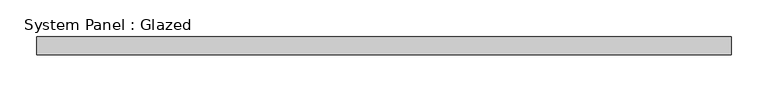
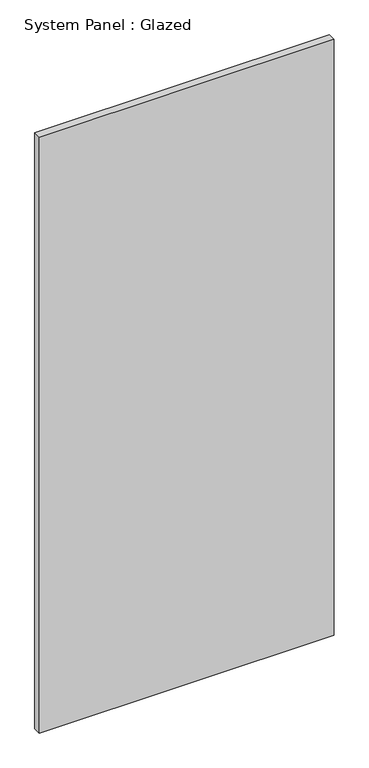
"""IFC4 building model written with IfcOpenShell, lengths in millimetres: plate geometry, System Panel : Glazed."""

from ifc_helpers import new_model, si_unit, origin, origin_with_axes, place, context, project, spatial, polyline, outline, extrude, source, transform, mapped, element, save


def system_panel_glazed_49f26875(model_context):
    return source(origin(), model_context, "Body", "SweptSolid", [
        extrude(outline(polyline([(475.0, 24.5), (-475.0, 24.5), (-475.0, 49.5), (475.0, 49.5), (475.0, 24.5)])), origin_with_axes(), (0.0, 0.0, 1.0), 2030.4462072),
    ])


if __name__ == "__main__":
    model = new_model("IFC4")
    model_context = context("Model", 3, world=origin())
    ifc_project = project(units=[si_unit("LENGTHUNIT", "METRE", prefix="MILLI")], contexts=[model_context])
    site = spatial("IfcSite", under=ifc_project)
    building = spatial("IfcBuilding", under=site)
    placement = place(None, origin())
    system_panel_glazed_shape = system_panel_glazed_49f26875(model_context)
    element("IfcPlate", 1, ObjectType="System Panel : Glazed", at=placement, inside=building, context=model_context, shape_type="MappedRepresentation", body=[
        mapped(system_panel_glazed_shape, transform((0.0, 0.0, 0.0), x_axis=(1.0, 0.0, 0.0), y_axis=(0.0, 1.0, 0.0), z_axis=(0.0, 0.0, 1.0))),
    ])
    save(model, "model.ifc")

# Revit data of these elements
# Type "System Panel : Glazed"
#   Construction Type Id = "GSP4R"
#   Analytic Construction = "1/8 in Pilkington single glazing"
#   Visual Light Transmittance = 0.9
#   Solar Heat Gain Coefficient = 0.86
#   Heat Transfer Coefficient (U) = 6.7069 W/(m²·K)
#   Define Thermal Properties by = 1
# Element 1 (IfcPlate, "System Panel : Glazed")
#   Materials on its faces: "Glass"
# Materials
#   "Glass": class "Glass", colour RGB 0 128 192, transparency 0.9, Description = "Soda Lime Glass", Cost = 0
